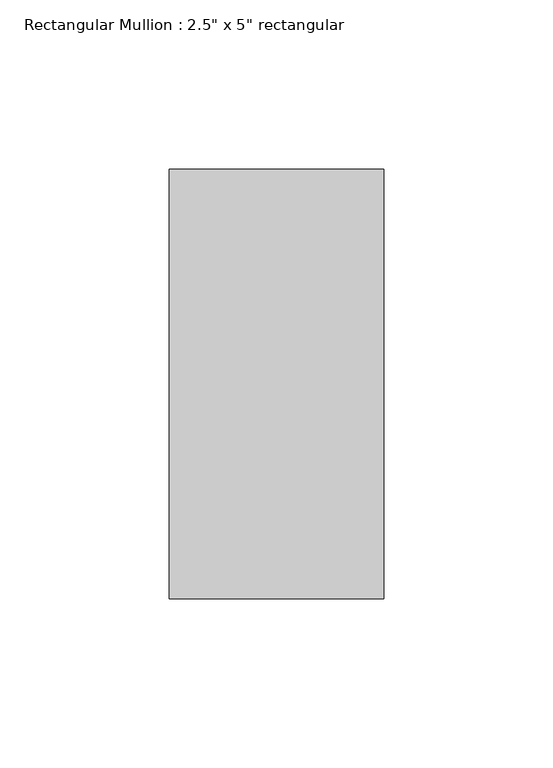
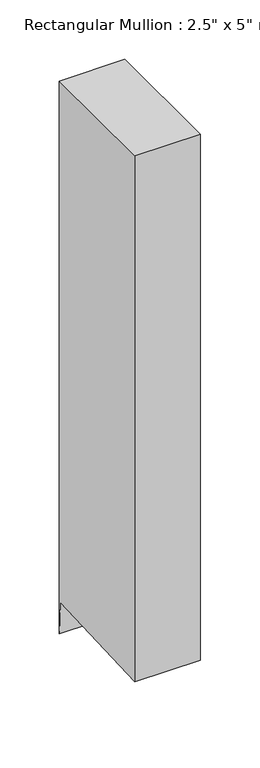
"""IFC4 building model written with IfcOpenShell, lengths in millimetres: member geometry."""

from ifc_helpers import new_model, si_unit, frame, origin, place, context, project, spatial, polyline, outline, extrude, source, transform, mapped, element, save


def member_dbd57660(model_context):
    return source(origin(), model_context, "Body", "SweptSolid", [
        extrude(outline(polyline([(-63.5, 0.0), (63.5, 0.0), (63.5, -568.018324), (62.0828234, -534.9390623), (-63.5, -540.3192622), (-63.5, 0.0)])), frame((-63.5, 0.0, 0.0), z_axis=(1.0, 0.0, 0.0), x_axis=(0.0, 1.0, 0.0)), (0.0, 0.0, 1.0), 63.5),
    ])


if __name__ == "__main__":
    model = new_model("IFC4")
    model_context = context("Model", 3, world=origin())
    ifc_project = project(units=[si_unit("LENGTHUNIT", "METRE", prefix="MILLI")], contexts=[model_context])
    site = spatial("IfcSite", under=ifc_project)
    building = spatial("IfcBuilding", under=site)
    placement = place(None, origin())
    member_shape = member_dbd57660(model_context)
    element("IfcMember", 1, ObjectType="Rectangular Mullion : 2.5\" x 5\" rectangular", at=placement, inside=building, context=model_context, shape_type="MappedRepresentation", body=[
        mapped(member_shape, transform((0.0, 0.0, 0.0), x_axis=(1.0, 0.0, 0.0), y_axis=(0.0, 1.0, 0.0), z_axis=(0.0, 0.0, 1.0))),
    ])
    save(model, "model.ifc")

# Revit data of these elements
# Type "Rectangular Mullion : 2.5\" x 5\" rectangular"
#   built-in parameter 1007304 = 0.416667 (stored number, unit not read)
#   built-in parameter 1007301 = 0.104167 (stored number, unit not read)
#   built-in parameter 1007300 = 0.104167 (stored number, unit not read)
# Element 1 (IfcMember, "Rectangular Mullion : 2.5\" x 5\" rectangular")
#   Materials on its faces: "Metal - Aluminum"
# Materials
#   "Metal - Aluminum": class "Metal", colour RGB 247 247 247, transparency 0, Cost = 0
